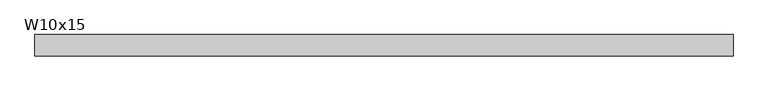
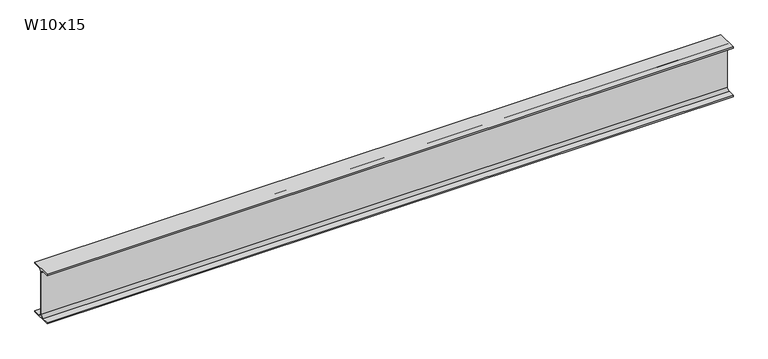
"""IFC4 building model written with IfcOpenShell, lengths in millimetres: beam geometry, RME W-Wide Flange : W10x15."""

from ifc_helpers import new_model, si_unit, point, frame, frame_2d, origin, place, context, project, spatial, polyline, circle_curve, trimmed, segment, composite_curve, outline, extrude, source, transform, mapped, element, save


def w10x15_0b83cb56(model_context):
    return source(origin(), model_context, "Body", "SweptSolid", [
        extrude(outline(composite_curve([segment(polyline([(50.8, -120.142), (50.8, -127.0), (-50.8, -127.0), (-50.8, -120.142), (-16.7005, -120.142)]), True, "CONTINUOUS"), segment(trimmed(circle_curve(frame_2d((-16.7005, -106.3625)), 13.7795), [point((-16.7005, -120.142))], [point((-2.921, -106.3625))], True, "CARTESIAN"), True, "CONTINUOUS"), segment(polyline([(-2.921, -106.3625), (-2.921, 106.3625)]), True, "CONTINUOUS"), segment(trimmed(circle_curve(frame_2d((-16.7005, 106.3625)), 13.7795), [point((-2.921, 106.3625))], [point((-16.7005, 120.142))], True, "CARTESIAN"), True, "CONTINUOUS"), segment(polyline([(-16.7005, 120.142), (-50.8, 120.142), (-50.8, 127.0), (50.8, 127.0), (50.8, 120.142), (16.7005, 120.142)]), True, "CONTINUOUS"), segment(trimmed(circle_curve(frame_2d((16.7005, 106.3625)), 13.7795), [point((16.7005, 120.142))], [point((2.921, 106.3625))], True, "CARTESIAN"), True, "CONTINUOUS"), segment(polyline([(2.921, 106.3625), (2.921, -106.3625)]), True, "CONTINUOUS"), segment(trimmed(circle_curve(frame_2d((16.7005, -106.3625)), 13.7795), [point((2.921, -106.3625))], [point((16.7005, -120.142))], True, "CARTESIAN"), True, "CONTINUOUS"), segment(polyline([(16.7005, -120.142), (50.8, -120.142)]), True, "CONTINUOUS")], self_intersect=False)), frame((-1655.9445644, 0.0, 0.0), z_axis=(1.0, 0.0, 0.0), x_axis=(0.0, 1.0, 0.0)), (0.0, 0.0, 1.0), 3311.8891289),
    ])


if __name__ == "__main__":
    model = new_model("IFC4")
    model_context = context("Model", 3, world=origin())
    ifc_project = project(units=[si_unit("LENGTHUNIT", "METRE", prefix="MILLI")], contexts=[model_context])
    site = spatial("IfcSite", under=ifc_project)
    building = spatial("IfcBuilding", under=site)
    placement = place(None, origin())
    w10x15_shape = w10x15_0b83cb56(model_context)
    element("IfcBeam", 1, ObjectType="RME W-Wide Flange : W10x15", at=placement, inside=building, context=model_context, shape_type="MappedRepresentation", body=[
        mapped(w10x15_shape, transform((0.0, 0.0, 0.0), x_axis=(1.0, 0.0, 0.0), y_axis=(0.0, 1.0, 0.0), z_axis=(0.0, 0.0, 1.0))),
    ])
    save(model, "model.ifc")

# Revit data of these elements
# Type "RME W-Wide Flange : W10x15"
#   WELD P [instance default] = ""
#   WELD LE [instance default] = ""
#   WELD D [instance default] = ""
#   TOP SECTION SIZE [instance default] = ""
#   TOP SECTION LENGTH [instance default] = ""
#   REMARKS [instance default] = ""
#   REINF TYPE [instance default] = ""
#   Nominal Size = "W24"
#   End Bearing Capacity [instance default] = ""
#   BOT SECTION SIZE [instance default] = ""
#   BOT SECTION LENGTH [instance default] = ""
#   Assembly Code = "B10"
#   W = 15
#   Start Extension Calculation [instance default] = 10' - 0"
#   Start Extension [instance default] = -0' - 0 1/2"
#   End Extension Calculation [instance default] = 10' - 0"
#   End Extension [instance default] = -0' - 0 1/2"
#   Length [instance default] = 5' - 0"
#   bf = 0' - 4"
#   d = 0' - 10"
#   k = 0' - 0 13/16"
#   k2 = 0' - 0.5425"
#   tf = 0' - 0.27"
#   tw = 0' - 0.23"
#   A = 0.030625 SF
#   Structural Material [instance default] = Metal - Steel - ASTM A992
# Element 1 (IfcBeam, "RME W-Wide Flange : W10x15")
#   Length = 10' - 10.38934"
#   Materials on its faces: "Metal - Steel - ASTM A992"
# Materials
#   "Metal - Steel - ASTM A992": class "Metal", colour RGB 255 128 0, transparency 0
